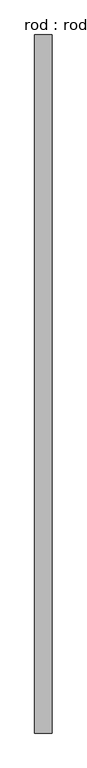
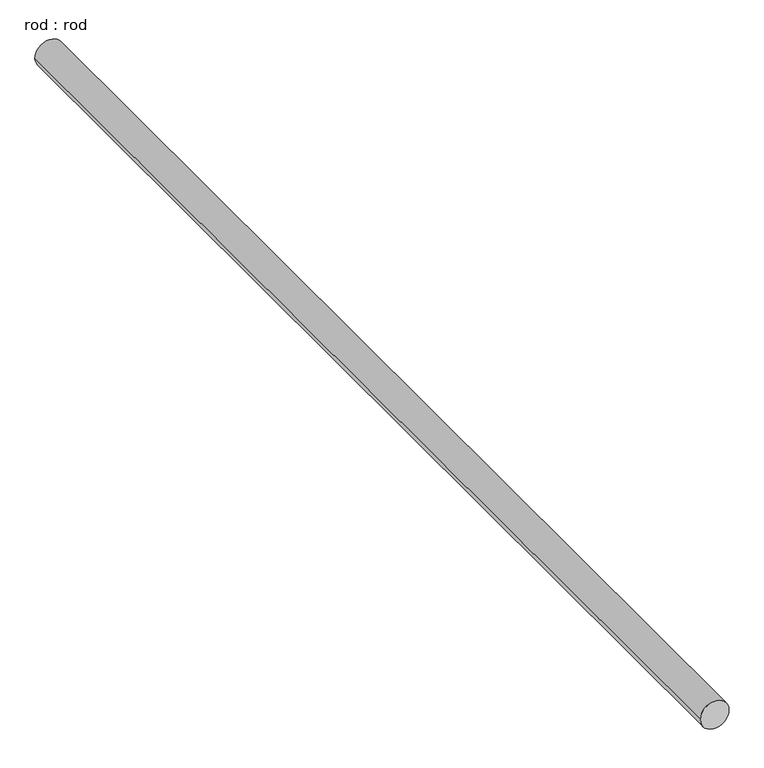
"""IFC4 building model written with IfcOpenShell, lengths in millimetres: proxy geometry, rod : rod."""

import ifcopenshell
import ifcopenshell.guid

model = None  # the IFC model being written
_history = None  # IfcOwnerHistory: only IFC2X3 demands one
_inside = {}  # id of a spatial element -> (the spatial element, [elements in it])
_under = {}  # id of a project, library or spatial element -> (it, [spatial elements below it])
_declared = {}  # id of a project -> (the project, [libraries it declares])
_typed = {}  # id of a type object -> (the type object, [elements of that type])
_made_of = {}  # id of a material, layer set ... -> (it, [elements and type objects made of it])


def new_model(schema):
    """Start an empty IFC model of exactly this schema.

    Asked for "IFC4X3", IfcOpenShell would pick the latest addendum, in which some entities
    have other attributes; the version numbers below select the first issue.
    IFC2X3 requires an IfcOwnerHistory on every rooted entity: one is made here for all.
    """
    global model, _history
    if schema == "IFC4X3":
        model = ifcopenshell.file(schema_version=(4, 3, 0, 0))
    else:
        model = ifcopenshell.file(schema=schema)
    _inside.clear()
    _under.clear()
    _declared.clear()
    _typed.clear()
    _made_of.clear()
    _history = None
    if model.schema == "IFC2X3":
        org = make("IfcOrganization", Name="unknown")
        user = make(
            "IfcPersonAndOrganization",
            ThePerson=make("IfcPerson", FamilyName="unknown"),
            TheOrganization=org,
        )
        app = make(
            "IfcApplication",
            ApplicationDeveloper=org,
            Version="unknown",
            ApplicationFullName="unknown",
            ApplicationIdentifier="unknown",
        )
        _history = make(
            "IfcOwnerHistory",
            OwningUser=user,
            OwningApplication=app,
            ChangeAction="ADDED",
            CreationDate=0,
        )
    return model


def make(cls, **values):
    """One entity of the class cls with the attributes given. An attribute that is None is left unset."""
    return model.create_entity(
        cls, **{name: value for name, value in values.items() if value is not None}
    )


def rooted(cls, **values):
    """An entity with a GlobalId (a new one), such as an element, a storey or a relation."""
    return make(cls, GlobalId=ifcopenshell.guid.new(), OwnerHistory=_history, **values)


def si_unit(unit_type, name, prefix=None):
    """IfcSIUnit, for example si_unit("LENGTHUNIT", "METRE", prefix="MILLI")."""
    return make("IfcSIUnit", UnitType=unit_type, Prefix=prefix, Name=name)


def assignment(units):
    """IfcUnitAssignment: the units of a project."""
    return None if units is None else make("IfcUnitAssignment", Units=units)


def point(xyz):
    """IfcCartesianPoint."""
    return None if xyz is None else make("IfcCartesianPoint", Coordinates=xyz)


def direction(xyz):
    """IfcDirection."""
    return None if xyz is None else make("IfcDirection", DirectionRatios=xyz)


def frame(location, z_axis=None, x_axis=None):
    """IfcAxis2Placement3D, a coordinate frame: its origin and axes. An axis left out is left unset."""
    return make(
        "IfcAxis2Placement3D",
        Location=point(location),
        Axis=direction(z_axis),
        RefDirection=direction(x_axis),
    )


def frame_2d(location, x_axis=None):
    """IfcAxis2Placement2D, a coordinate frame in the plane: its origin and x axis."""
    return make(
        "IfcAxis2Placement2D", Location=point(location), RefDirection=direction(x_axis)
    )


def origin():
    """The frame at (0, 0, 0) with its axes left unset."""
    return frame((0.0, 0.0, 0.0))


def place(relative_to, where):
    """IfcLocalPlacement: puts the frame where relative to a parent placement (None: the world)."""
    return make(
        "IfcLocalPlacement", PlacementRelTo=relative_to, RelativePlacement=where
    )


def context(
    kind, dimensions, precision=None, world=None, true_north=None, identifier=None
):
    """IfcGeometricRepresentationContext, for example the 3D "Model" context."""
    return make(
        "IfcGeometricRepresentationContext",
        ContextIdentifier=identifier,
        ContextType=kind,
        CoordinateSpaceDimension=dimensions,
        Precision=precision,
        WorldCoordinateSystem=world,
        TrueNorth=true_north,
    )


def project(units=None, contexts=None):
    """IfcProject with its units and contexts."""
    return rooted(
        "IfcProject",
        Name="project",
        RepresentationContexts=contexts,
        UnitsInContext=assignment(units),
    )


def spatial(cls, under=None, at=None, **own):
    """A site, building, storey or space (cls), placed at a placement, below another one or the project."""
    s = rooted(cls, ObjectPlacement=at, **own)
    if under is not None:
        _under.setdefault(under.id(), (under, []))[1].append(s)
    return s


def circle_curve(where, radius):
    """IfcCircle in the frame where."""
    return make("IfcCircle", Position=where, Radius=radius)


def trimmed(basis, trim1, trim2, sense, master):
    """IfcTrimmedCurve: the piece of a basis curve between two trims."""
    return make(
        "IfcTrimmedCurve",
        BasisCurve=basis,
        Trim1=trim1,
        Trim2=trim2,
        SenseAgreement=sense,
        MasterRepresentation=master,
    )


def segment(curve, same_sense, transition):
    """IfcCompositeCurveSegment."""
    return make(
        "IfcCompositeCurveSegment",
        Transition=transition,
        SameSense=same_sense,
        ParentCurve=curve,
    )


def composite_curve(segments, self_intersect=None):
    """IfcCompositeCurve: segments joined end to end."""
    return make("IfcCompositeCurve", Segments=segments, SelfIntersect=self_intersect)


def outline(outer, holes=None, kind="AREA"):
    """IfcArbitraryClosedProfileDef: a profile drawn as a closed curve; with holes, ...WithVoids."""
    if holes is None:
        return make("IfcArbitraryClosedProfileDef", ProfileType=kind, OuterCurve=outer)
    return make(
        "IfcArbitraryProfileDefWithVoids",
        ProfileType=kind,
        OuterCurve=outer,
        InnerCurves=holes,
    )


def extrude(swept, where, along, depth):
    """IfcExtrudedAreaSolid: the profile swept, set in the frame where, extruded along a direction by depth."""
    return make(
        "IfcExtrudedAreaSolid",
        SweptArea=swept,
        Position=where,
        ExtrudedDirection=direction(along),
        Depth=depth,
    )


def shape(context_of_items, identifier, shape_type, items):
    """IfcShapeRepresentation: the items that make up one representation, for example the "Body"."""
    return make(
        "IfcShapeRepresentation",
        ContextOfItems=context_of_items,
        RepresentationIdentifier=identifier,
        RepresentationType=shape_type,
        Items=items,
    )


def source(mapping_origin, context_of_items, identifier, shape_type, items):
    """IfcRepresentationMap: a shape defined once, which mapped items show again and again."""
    return make(
        "IfcRepresentationMap",
        MappingOrigin=mapping_origin,
        MappedRepresentation=shape(context_of_items, identifier, shape_type, items),
    )


def transform(
    local_origin,
    x_axis=None,
    y_axis=None,
    z_axis=None,
    scale=None,
    scale2=None,
    scale3=None,
    uniform=True,
):
    """IfcCartesianTransformationOperator3D, or its non-uniform kind. x_axis, y_axis, z_axis: its Axis1, 2, 3."""
    if uniform:
        return make(
            "IfcCartesianTransformationOperator3D",
            Axis1=direction(x_axis),
            Axis2=direction(y_axis),
            LocalOrigin=point(local_origin),
            Scale=scale,
            Axis3=direction(z_axis),
        )
    return make(
        "IfcCartesianTransformationOperator3DnonUniform",
        Axis1=direction(x_axis),
        Axis2=direction(y_axis),
        LocalOrigin=point(local_origin),
        Scale=scale,
        Axis3=direction(z_axis),
        Scale2=scale2,
        Scale3=scale3,
    )


def mapped(mapping_source, mapping_target):
    """IfcMappedItem: shows the shape of a source again, moved by a transform."""
    return make(
        "IfcMappedItem", MappingSource=mapping_source, MappingTarget=mapping_target
    )


def made_of(thing, what):
    """Note that an element or type object is made of a material, layer set ...; save() writes the relation."""
    if what is not None:
        _made_of.setdefault(what.id(), (what, []))[1].append(thing)
    return thing


def element(
    cls,
    number,
    at=None,
    inside=None,
    cuts=None,
    type_object=None,
    material=None,
    context=None,
    identifier="Body",
    shape_type=None,
    held_by="IfcProductDefinitionShape",
    body=None,
    shapes=None,
    **own,
):
    """One element of the class cls, such as IfcWall. Its Tag is "e" and its number.

    at: its placement. inside: the storey or other place that contains it. cuts: it is an
    opening in that element (IfcRelVoidsElement). A single representation is given by context,
    identifier, shape_type and body (its items); several are given by shapes. held_by: the class
    of the entity that holds the representations. save() writes the other relations.
    """
    e = rooted(cls, Tag="e%d" % number, ObjectPlacement=at, **own)
    if body is not None:
        shapes = [shape(context, identifier, shape_type, body)]
    if shapes is not None:
        e.Representation = make(held_by, Representations=shapes)
    if inside is not None:
        _inside.setdefault(inside.id(), (inside, []))[1].append(e)
    if cuts is not None:
        rooted(
            "IfcRelVoidsElement", RelatingBuildingElement=cuts, RelatedOpeningElement=e
        )
    if type_object is not None:
        _typed.setdefault(type_object.id(), (type_object, []))[1].append(e)
    return made_of(e, material)


def aggregate(whole, parts):
    """IfcRelAggregates: a whole, such as a stair, and the parts it consists of."""
    return rooted("IfcRelAggregates", RelatingObject=whole, RelatedObjects=parts)


def save(model, path):
    """Write the relations noted so far, then the file.

    IfcRelAggregates (storeys below a building ...), IfcRelContainedInSpatialStructure (elements
    in a storey), IfcRelDefinesByType, IfcRelAssociatesMaterial and IfcRelDeclares: one each for
    every whole, place, type object, material and project.
    """
    for whole, parts in _under.values():
        aggregate(whole, parts)
    for where, things in _inside.values():
        rooted(
            "IfcRelContainedInSpatialStructure",
            RelatedElements=things,
            RelatingStructure=where,
        )
    for kind, things in _typed.values():
        rooted("IfcRelDefinesByType", RelatedObjects=things, RelatingType=kind)
    for what, things in _made_of.values():
        rooted("IfcRelAssociatesMaterial", RelatedObjects=things, RelatingMaterial=what)
    for by, libraries in _declared.values():
        rooted("IfcRelDeclares", RelatingContext=by, RelatedDefinitions=libraries)
    model.write(path)


def rod_rod_9103a248(model_context):
    return source(origin(), model_context, "Body", "SweptSolid", [
        extrude(outline(composite_curve([segment(trimmed(circle_curve(frame_2d((0.0108462, 0.0)), 200.0), [point((0.0108462, 200.0))], [point((0.0108462, -200.0))], False, "CARTESIAN"), True, "CONTINUOUS"), segment(trimmed(circle_curve(frame_2d((0.0108462, 0.0)), 200.0), [point((0.0108462, -200.0))], [point((0.0108462, 200.0))], False, "CARTESIAN"), True, "CONTINUOUS")], self_intersect=False)), frame((0.0, -3929.5928132, 0.0), z_axis=(0.0, 1.0, 0.0), x_axis=(0.0, 0.0, 1.0)), (0.0, 0.0, 1.0), 16044.6428571),
    ])


if __name__ == "__main__":
    model = new_model("IFC4")
    model_context = context("Model", 3, world=origin())
    ifc_project = project(units=[si_unit("LENGTHUNIT", "METRE", prefix="MILLI")], contexts=[model_context])
    site = spatial("IfcSite", under=ifc_project)
    building = spatial("IfcBuilding", under=site)
    placement = place(None, origin())
    rod_rod_shape = rod_rod_9103a248(model_context)
    element("IfcBuildingElementProxy", 1, Name="rod : rod", ObjectType="rod : rod", at=placement, inside=building, context=model_context, shape_type="MappedRepresentation", body=[
        mapped(rod_rod_shape, transform((0.0, 0.0, 0.0), x_axis=(1.0, 0.0, 0.0), y_axis=(0.0, 1.0, 0.0), z_axis=(0.0, 0.0, 1.0))),
    ])
    save(model, "model.ifc")

# Revit data of these elements
# Type "rod : rod"
#   Default Elevation = 0
